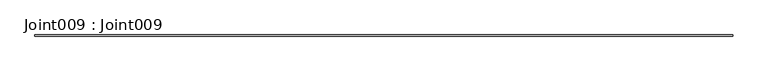
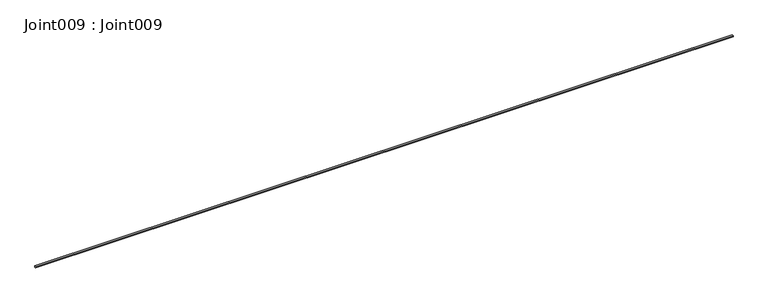
"""IFC4 building model written with IfcOpenShell, lengths in millimetres: proxy geometry, Joint009 : Joint009."""

from ifc_helpers import new_model, si_unit, point, frame, frame_2d, origin, place, context, project, spatial, polyline, circle_curve, trimmed, segment, composite_curve, outline, extrude, source, transform, mapped, element, save


def joint009_joint009_4a87faaf(model_context):
    return source(origin(), model_context, "Body", "SweptSolid", [
        extrude(outline(composite_curve([segment(polyline([(-4376.7836914, 42587.1101563), (-4376.7836914, 42583.1921875)]), True, "CONTINUOUS"), segment(trimmed(circle_curve(frame_2d((-4378.3820234, 42578.0203125)), 5.4132205), [point((-4376.7836914, 42583.1921875))], [point((-4379.9803555, 42583.1921875))], True, "CARTESIAN"), True, "CONTINUOUS"), segment(polyline([(-4379.9803555, 42583.1921875), (-4379.9803555, 42587.1101563)]), True, "CONTINUOUS"), segment(trimmed(circle_curve(frame_2d((-4378.3820234, 42581.9382813)), 5.4132205), [point((-4379.9803555, 42587.1101563))], [point((-4376.7836914, 42587.1101563))], False, "CARTESIAN"), True, "CONTINUOUS")], self_intersect=False)), frame((12383.0178845, 0.0, 0.0), z_axis=(1.0, 0.0, 0.0), x_axis=(0.0, 1.0, 0.0)), (0.0, 0.0, 1.0), 2000.0),
    ])


if __name__ == "__main__":
    model = new_model("IFC4")
    model_context = context("Model", 3, world=origin())
    ifc_project = project(units=[si_unit("LENGTHUNIT", "METRE", prefix="MILLI")], contexts=[model_context])
    site = spatial("IfcSite", under=ifc_project)
    building = spatial("IfcBuilding", under=site)
    placement = place(None, origin())
    joint009_joint009_shape = joint009_joint009_4a87faaf(model_context)
    element("IfcBuildingElementProxy", 1, Name="Joint009 : Joint009", ObjectType="Joint009 : Joint009", at=placement, inside=building, context=model_context, shape_type="MappedRepresentation", body=[
        mapped(joint009_joint009_shape, transform((0.0, 0.0, 0.0), x_axis=(1.0, 0.0, 0.0), y_axis=(0.0, 1.0, 0.0), z_axis=(0.0, 0.0, 1.0))),
    ])
    save(model, "model.ifc")

# Revit data of these elements
# Type "Joint009 : Joint009"
#   NameOverride = "Joint009"
# Element 1 (IfcBuildingElementProxy, "Joint009 : Joint009")
#   Materials on its faces: "SILICON JOINT"
# Materials
#   "SILICON JOINT": class "Unassigned", colour RGB 150 184 127, transparency 0
